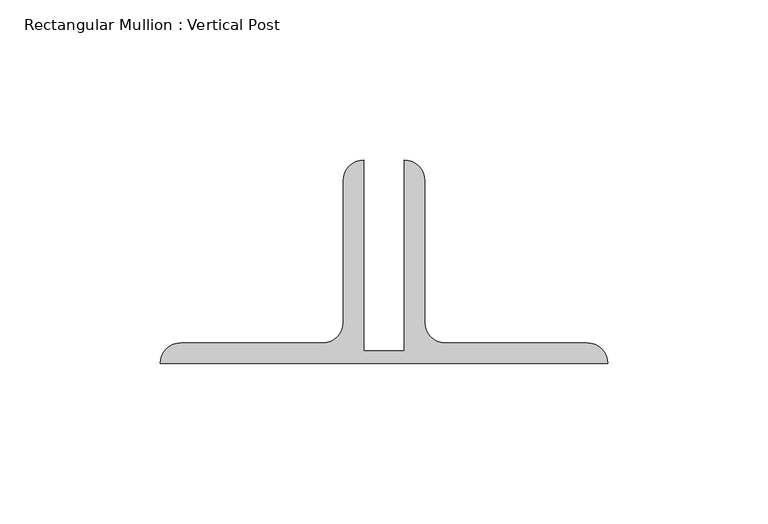
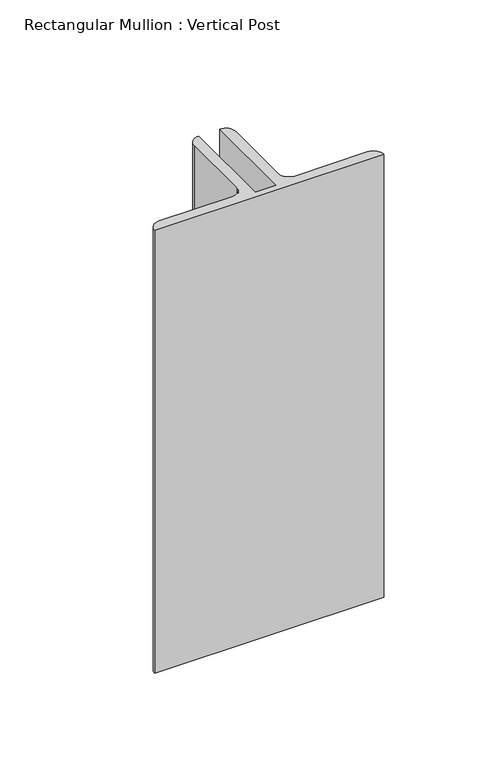
"""IFC4 building model written with IfcOpenShell, lengths in millimetres: member geometry, Rectangular Mullion : Vertical Post."""

import ifcopenshell
import ifcopenshell.guid

model = None  # the IFC model being written
_history = None  # IfcOwnerHistory: only IFC2X3 demands one
_inside = {}  # id of a spatial element -> (the spatial element, [elements in it])
_under = {}  # id of a project, library or spatial element -> (it, [spatial elements below it])
_declared = {}  # id of a project -> (the project, [libraries it declares])
_typed = {}  # id of a type object -> (the type object, [elements of that type])
_made_of = {}  # id of a material, layer set ... -> (it, [elements and type objects made of it])


def new_model(schema):
    """Start an empty IFC model of exactly this schema.

    Asked for "IFC4X3", IfcOpenShell would pick the latest addendum, in which some entities
    have other attributes; the version numbers below select the first issue.
    IFC2X3 requires an IfcOwnerHistory on every rooted entity: one is made here for all.
    """
    global model, _history
    if schema == "IFC4X3":
        model = ifcopenshell.file(schema_version=(4, 3, 0, 0))
    else:
        model = ifcopenshell.file(schema=schema)
    _inside.clear()
    _under.clear()
    _declared.clear()
    _typed.clear()
    _made_of.clear()
    _history = None
    if model.schema == "IFC2X3":
        org = make("IfcOrganization", Name="unknown")
        user = make(
            "IfcPersonAndOrganization",
            ThePerson=make("IfcPerson", FamilyName="unknown"),
            TheOrganization=org,
        )
        app = make(
            "IfcApplication",
            ApplicationDeveloper=org,
            Version="unknown",
            ApplicationFullName="unknown",
            ApplicationIdentifier="unknown",
        )
        _history = make(
            "IfcOwnerHistory",
            OwningUser=user,
            OwningApplication=app,
            ChangeAction="ADDED",
            CreationDate=0,
        )
    return model


def make(cls, **values):
    """One entity of the class cls with the attributes given. An attribute that is None is left unset."""
    return model.create_entity(
        cls, **{name: value for name, value in values.items() if value is not None}
    )


def rooted(cls, **values):
    """An entity with a GlobalId (a new one), such as an element, a storey or a relation."""
    return make(cls, GlobalId=ifcopenshell.guid.new(), OwnerHistory=_history, **values)


def si_unit(unit_type, name, prefix=None):
    """IfcSIUnit, for example si_unit("LENGTHUNIT", "METRE", prefix="MILLI")."""
    return make("IfcSIUnit", UnitType=unit_type, Prefix=prefix, Name=name)


def assignment(units):
    """IfcUnitAssignment: the units of a project."""
    return None if units is None else make("IfcUnitAssignment", Units=units)


def point(xyz):
    """IfcCartesianPoint."""
    return None if xyz is None else make("IfcCartesianPoint", Coordinates=xyz)


def direction(xyz):
    """IfcDirection."""
    return None if xyz is None else make("IfcDirection", DirectionRatios=xyz)


def frame(location, z_axis=None, x_axis=None):
    """IfcAxis2Placement3D, a coordinate frame: its origin and axes. An axis left out is left unset."""
    return make(
        "IfcAxis2Placement3D",
        Location=point(location),
        Axis=direction(z_axis),
        RefDirection=direction(x_axis),
    )


def frame_2d(location, x_axis=None):
    """IfcAxis2Placement2D, a coordinate frame in the plane: its origin and x axis."""
    return make(
        "IfcAxis2Placement2D", Location=point(location), RefDirection=direction(x_axis)
    )


def origin():
    """The frame at (0, 0, 0) with its axes left unset."""
    return frame((0.0, 0.0, 0.0))


def place(relative_to, where):
    """IfcLocalPlacement: puts the frame where relative to a parent placement (None: the world)."""
    return make(
        "IfcLocalPlacement", PlacementRelTo=relative_to, RelativePlacement=where
    )


def context(
    kind, dimensions, precision=None, world=None, true_north=None, identifier=None
):
    """IfcGeometricRepresentationContext, for example the 3D "Model" context."""
    return make(
        "IfcGeometricRepresentationContext",
        ContextIdentifier=identifier,
        ContextType=kind,
        CoordinateSpaceDimension=dimensions,
        Precision=precision,
        WorldCoordinateSystem=world,
        TrueNorth=true_north,
    )


def project(units=None, contexts=None):
    """IfcProject with its units and contexts."""
    return rooted(
        "IfcProject",
        Name="project",
        RepresentationContexts=contexts,
        UnitsInContext=assignment(units),
    )


def spatial(cls, under=None, at=None, **own):
    """A site, building, storey or space (cls), placed at a placement, below another one or the project."""
    s = rooted(cls, ObjectPlacement=at, **own)
    if under is not None:
        _under.setdefault(under.id(), (under, []))[1].append(s)
    return s


def polyline(points):
    """IfcPolyline through the points."""
    return make("IfcPolyline", Points=[point(p) for p in points])


def circle_curve(where, radius):
    """IfcCircle in the frame where."""
    return make("IfcCircle", Position=where, Radius=radius)


def trimmed(basis, trim1, trim2, sense, master):
    """IfcTrimmedCurve: the piece of a basis curve between two trims."""
    return make(
        "IfcTrimmedCurve",
        BasisCurve=basis,
        Trim1=trim1,
        Trim2=trim2,
        SenseAgreement=sense,
        MasterRepresentation=master,
    )


def segment(curve, same_sense, transition):
    """IfcCompositeCurveSegment."""
    return make(
        "IfcCompositeCurveSegment",
        Transition=transition,
        SameSense=same_sense,
        ParentCurve=curve,
    )


def composite_curve(segments, self_intersect=None):
    """IfcCompositeCurve: segments joined end to end."""
    return make("IfcCompositeCurve", Segments=segments, SelfIntersect=self_intersect)


def outline(outer, holes=None, kind="AREA"):
    """IfcArbitraryClosedProfileDef: a profile drawn as a closed curve; with holes, ...WithVoids."""
    if holes is None:
        return make("IfcArbitraryClosedProfileDef", ProfileType=kind, OuterCurve=outer)
    return make(
        "IfcArbitraryProfileDefWithVoids",
        ProfileType=kind,
        OuterCurve=outer,
        InnerCurves=holes,
    )


def extrude(swept, where, along, depth):
    """IfcExtrudedAreaSolid: the profile swept, set in the frame where, extruded along a direction by depth."""
    return make(
        "IfcExtrudedAreaSolid",
        SweptArea=swept,
        Position=where,
        ExtrudedDirection=direction(along),
        Depth=depth,
    )


def shape(context_of_items, identifier, shape_type, items):
    """IfcShapeRepresentation: the items that make up one representation, for example the "Body"."""
    return make(
        "IfcShapeRepresentation",
        ContextOfItems=context_of_items,
        RepresentationIdentifier=identifier,
        RepresentationType=shape_type,
        Items=items,
    )


def source(mapping_origin, context_of_items, identifier, shape_type, items):
    """IfcRepresentationMap: a shape defined once, which mapped items show again and again."""
    return make(
        "IfcRepresentationMap",
        MappingOrigin=mapping_origin,
        MappedRepresentation=shape(context_of_items, identifier, shape_type, items),
    )


def transform(
    local_origin,
    x_axis=None,
    y_axis=None,
    z_axis=None,
    scale=None,
    scale2=None,
    scale3=None,
    uniform=True,
):
    """IfcCartesianTransformationOperator3D, or its non-uniform kind. x_axis, y_axis, z_axis: its Axis1, 2, 3."""
    if uniform:
        return make(
            "IfcCartesianTransformationOperator3D",
            Axis1=direction(x_axis),
            Axis2=direction(y_axis),
            LocalOrigin=point(local_origin),
            Scale=scale,
            Axis3=direction(z_axis),
        )
    return make(
        "IfcCartesianTransformationOperator3DnonUniform",
        Axis1=direction(x_axis),
        Axis2=direction(y_axis),
        LocalOrigin=point(local_origin),
        Scale=scale,
        Axis3=direction(z_axis),
        Scale2=scale2,
        Scale3=scale3,
    )


def mapped(mapping_source, mapping_target):
    """IfcMappedItem: shows the shape of a source again, moved by a transform."""
    return make(
        "IfcMappedItem", MappingSource=mapping_source, MappingTarget=mapping_target
    )


def made_of(thing, what):
    """Note that an element or type object is made of a material, layer set ...; save() writes the relation."""
    if what is not None:
        _made_of.setdefault(what.id(), (what, []))[1].append(thing)
    return thing


def element(
    cls,
    number,
    at=None,
    inside=None,
    cuts=None,
    type_object=None,
    material=None,
    context=None,
    identifier="Body",
    shape_type=None,
    held_by="IfcProductDefinitionShape",
    body=None,
    shapes=None,
    **own,
):
    """One element of the class cls, such as IfcWall. Its Tag is "e" and its number.

    at: its placement. inside: the storey or other place that contains it. cuts: it is an
    opening in that element (IfcRelVoidsElement). A single representation is given by context,
    identifier, shape_type and body (its items); several are given by shapes. held_by: the class
    of the entity that holds the representations. save() writes the other relations.
    """
    e = rooted(cls, Tag="e%d" % number, ObjectPlacement=at, **own)
    if body is not None:
        shapes = [shape(context, identifier, shape_type, body)]
    if shapes is not None:
        e.Representation = make(held_by, Representations=shapes)
    if inside is not None:
        _inside.setdefault(inside.id(), (inside, []))[1].append(e)
    if cuts is not None:
        rooted(
            "IfcRelVoidsElement", RelatingBuildingElement=cuts, RelatedOpeningElement=e
        )
    if type_object is not None:
        _typed.setdefault(type_object.id(), (type_object, []))[1].append(e)
    return made_of(e, material)


def aggregate(whole, parts):
    """IfcRelAggregates: a whole, such as a stair, and the parts it consists of."""
    return rooted("IfcRelAggregates", RelatingObject=whole, RelatedObjects=parts)


def save(model, path):
    """Write the relations noted so far, then the file.

    IfcRelAggregates (storeys below a building ...), IfcRelContainedInSpatialStructure (elements
    in a storey), IfcRelDefinesByType, IfcRelAssociatesMaterial and IfcRelDeclares: one each for
    every whole, place, type object, material and project.
    """
    for whole, parts in _under.values():
        aggregate(whole, parts)
    for where, things in _inside.values():
        rooted(
            "IfcRelContainedInSpatialStructure",
            RelatedElements=things,
            RelatingStructure=where,
        )
    for kind, things in _typed.values():
        rooted("IfcRelDefinesByType", RelatedObjects=things, RelatingType=kind)
    for what, things in _made_of.values():
        rooted("IfcRelAssociatesMaterial", RelatedObjects=things, RelatingMaterial=what)
    for by, libraries in _declared.values():
        rooted("IfcRelDeclares", RelatingContext=by, RelatedDefinitions=libraries)
    model.write(path)


def rectangular_mullion_vertical_post_240526a2(model_context):
    return source(origin(), model_context, "Body", "SweptSolid", [
        extrude(outline(composite_curve([segment(polyline([(-6.35, 22.9145205), (6.35, 22.9145205), (6.35, 82.55)]), True, "CONTINUOUS"), segment(trimmed(circle_curve(frame_2d((6.35, 76.2)), 6.35), [point((6.35, 82.55))], [point((12.7, 76.2))], False, "CARTESIAN"), True, "CONTINUOUS"), segment(polyline([(12.7, 76.2), (12.7, 31.75)]), True, "CONTINUOUS"), segment(trimmed(circle_curve(frame_2d((19.05, 31.75)), 6.35), [point((12.7, 31.75))], [point((19.05, 25.4))], True, "CARTESIAN"), True, "CONTINUOUS"), segment(polyline([(19.05, 25.4), (63.5, 25.4)]), True, "CONTINUOUS"), segment(trimmed(circle_curve(frame_2d((63.5, 19.05)), 6.35), [point((63.5, 25.4))], [point((69.85, 19.05))], False, "CARTESIAN"), True, "CONTINUOUS"), segment(polyline([(69.85, 19.05), (-69.85, 19.05)]), True, "CONTINUOUS"), segment(trimmed(circle_curve(frame_2d((-63.5, 19.05)), 6.35), [point((-69.85, 19.05))], [point((-63.5, 25.4))], False, "CARTESIAN"), True, "CONTINUOUS"), segment(polyline([(-63.5, 25.4), (-19.05, 25.4)]), True, "CONTINUOUS"), segment(trimmed(circle_curve(frame_2d((-19.05, 31.75)), 6.35), [point((-19.05, 25.4))], [point((-12.7, 31.75))], True, "CARTESIAN"), True, "CONTINUOUS"), segment(polyline([(-12.7, 31.75), (-12.7, 76.2)]), True, "CONTINUOUS"), segment(trimmed(circle_curve(frame_2d((-6.35, 76.2)), 6.35), [point((-12.7, 76.2))], [point((-6.35, 82.55))], False, "CARTESIAN"), True, "CONTINUOUS"), segment(polyline([(-6.35, 82.55), (-6.35, 22.9145205)]), True, "CONTINUOUS")], self_intersect=False)), frame((0.0, 0.0, -285.5889998), z_axis=(0.0, 0.0, 1.0), x_axis=(1.0, 0.0, 0.0)), (0.0, 0.0, 1.0), 285.5889998),
    ])


if __name__ == "__main__":
    model = new_model("IFC4")
    model_context = context("Model", 3, world=origin())
    ifc_project = project(units=[si_unit("LENGTHUNIT", "METRE", prefix="MILLI")], contexts=[model_context])
    site = spatial("IfcSite", under=ifc_project)
    building = spatial("IfcBuilding", under=site)
    placement = place(None, origin())
    rectangular_mullion_vertical_post_shape = rectangular_mullion_vertical_post_240526a2(model_context)
    element("IfcMember", 1, ObjectType="Rectangular Mullion : Vertical Post", at=placement, inside=building, context=model_context, shape_type="MappedRepresentation", body=[
        mapped(rectangular_mullion_vertical_post_shape, transform((0.0, 0.0, 0.0), x_axis=(1.0, 0.0, 0.0), y_axis=(0.0, 1.0, 0.0), z_axis=(0.0, 0.0, 1.0))),
    ])
    save(model, "model.ifc")

# Revit data of these elements
# Type "Rectangular Mullion : Vertical Post"
#   built-in parameter 1007351 = -0.0625 (stored number, unit not read)
#   built-in parameter 1007322 = 0.0126789 (stored number, unit not read)
#   built-in parameter 1007321 = 0.229167 (stored number, unit not read)
#   built-in parameter 1007320 = 0.229167 (stored number, unit not read)
# Element 1 (IfcMember, "Rectangular Mullion : Vertical Post")
#   Materials on its faces: "GATE POST: GALVANIZED ANGLES"
# Materials
#   "GATE POST: GALVANIZED ANGLES": class "Unassigned", colour RGB 120 120 120, transparency 0, Cost = 0
